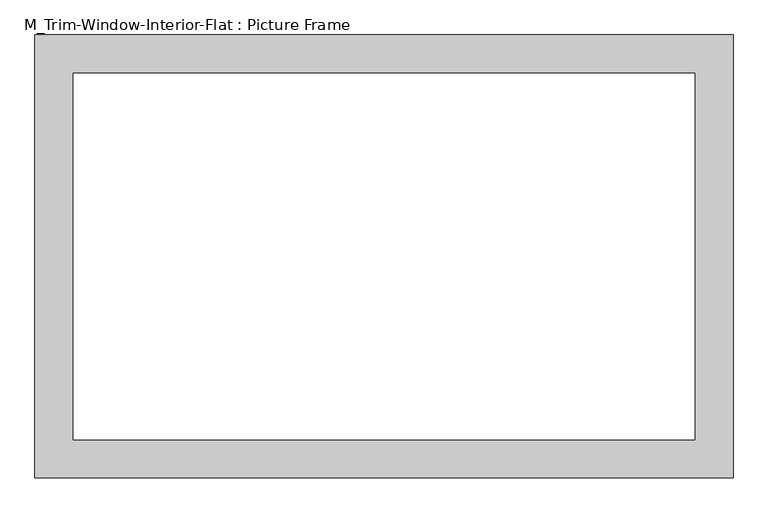
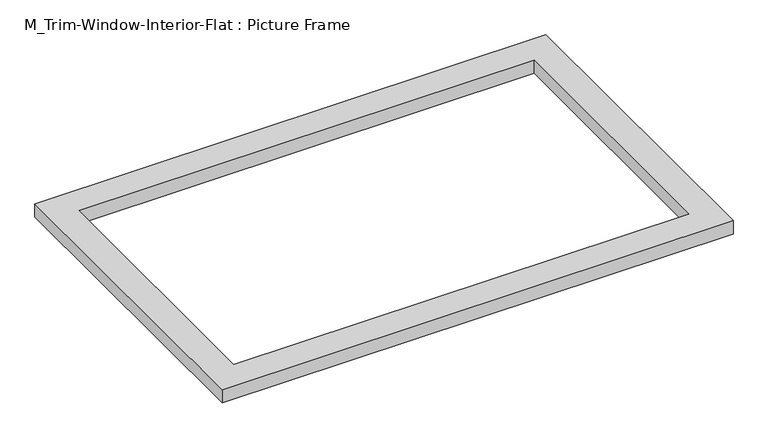
"""IFC4 building model written with IfcOpenShell, lengths in millimetres: proxy geometry, M_Trim-Window-Interior-Flat : Picture Frame."""

from ifc_helpers import new_model, si_unit, origin, origin_with_axes, place, context, project, spatial, polyline, outline, extrude, source, transform, mapped, element, save


def m_trim_window_interior_flat_picture_frame_3aaabd9e(model_context):
    return source(origin(), model_context, "Body", "SweptSolid", [
        extrude(outline(polyline([(547.3, 47.3), (547.3, -647.3), (-547.3, -647.3), (-547.3, 47.3), (547.3, 47.3)]), holes=[polyline([(487.3, -12.7), (-487.3, -12.7), (-487.3, -587.3), (487.3, -587.3), (487.3, -12.7)])]), origin_with_axes(), (0.0, 0.0, 1.0), 30.0),
    ])


if __name__ == "__main__":
    model = new_model("IFC4")
    model_context = context("Model", 3, world=origin())
    ifc_project = project(units=[si_unit("LENGTHUNIT", "METRE", prefix="MILLI")], contexts=[model_context])
    site = spatial("IfcSite", under=ifc_project)
    building = spatial("IfcBuilding", under=site)
    placement = place(None, origin())
    m_trim_window_interior_flat_picture_frame_shape = m_trim_window_interior_flat_picture_frame_3aaabd9e(model_context)
    element("IfcBuildingElementProxy", 1, Name="M_Trim-Window-Interior-Flat : Picture Frame", ObjectType="M_Trim-Window-Interior-Flat : Picture Frame", at=placement, inside=building, context=model_context, shape_type="MappedRepresentation", body=[
        mapped(m_trim_window_interior_flat_picture_frame_shape, transform((0.0, 0.0, 0.0), x_axis=(1.0, 0.0, 0.0), y_axis=(0.0, 1.0, 0.0), z_axis=(0.0, 0.0, 1.0))),
    ])
    save(model, "model.ifc")

# Revit data of these elements
# Type "M_Trim-Window-Interior-Flat : Picture Frame"
#   Trim Thickness_Picture Frame = 30 mm
#   Trim Width = 60 mm
#   Trim Thickness_with Sill = 20 mm
#   Sill Thickness = 30 mm
#   Opening Width [instance default] = 600 mm
#   Opening Height [instance default] = 900 mm
#   Default Elevation = 1200 mm
#   Sill = no
#   Picture Frame = yes
#   Trim Material [instance default] = none
# Element 1 (IfcBuildingElementProxy, "M_Trim-Window-Interior-Flat : Picture Frame")
#   Opening Width = 1000 mm
#   Opening Height = 600 mm
#   Trim Material = Wood - Stained
#   Materials on its faces: "Wood - Stained"
# Materials
#   "Wood - Stained": class "Wood", colour RGB 173 132 96, transparency 0, Cost = 0
